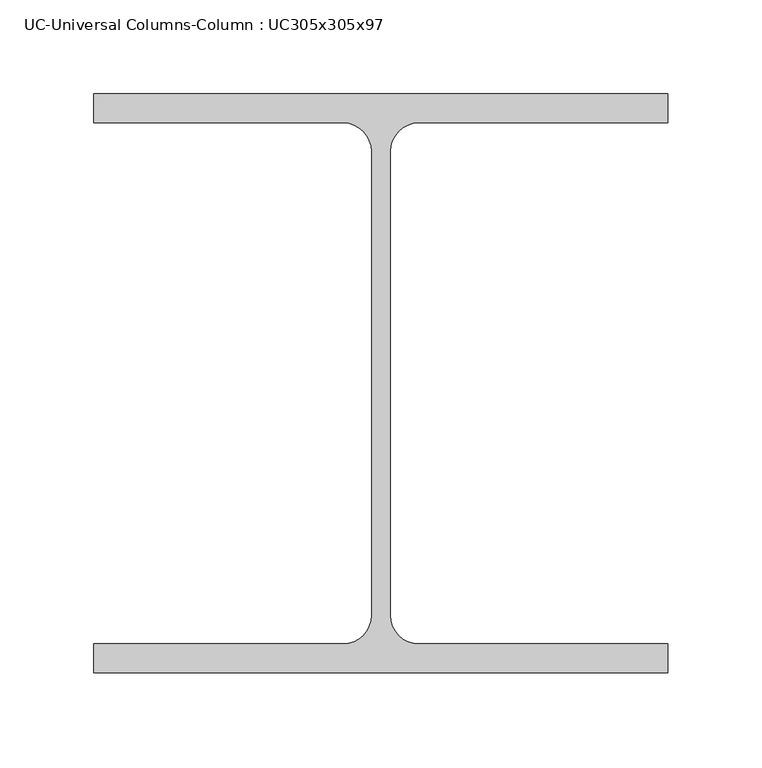
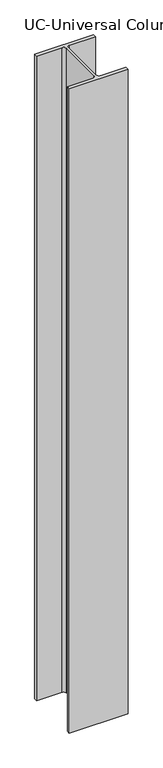
"""IFC4 building model written with IfcOpenShell, lengths in millimetres: column geometry, UC-Universal Columns-Column : UC305x305x97."""

from ifc_helpers import new_model, si_unit, point, frame_2d, origin, origin_with_axes, place, context, project, spatial, polyline, circle_curve, trimmed, segment, composite_curve, outline, extrude, source, transform, mapped, element, save


def uc_universal_columns_column_uc305x305x97_78c6f2b7(model_context):
    return source(origin(), model_context, "Body", "SweptSolid", [
        extrude(outline(composite_curve([segment(polyline([(152.65, -153.95), (-152.65, -153.95), (-152.65, -138.55), (-20.15, -138.55)]), True, "CONTINUOUS"), segment(trimmed(circle_curve(frame_2d((-20.15, -123.35)), 15.2), [point((-20.15, -138.55))], [point((-4.95, -123.35))], True, "CARTESIAN"), True, "CONTINUOUS"), segment(polyline([(-4.95, -123.35), (-4.95, 123.35)]), True, "CONTINUOUS"), segment(trimmed(circle_curve(frame_2d((-20.15, 123.35)), 15.2), [point((-4.95, 123.35))], [point((-20.15, 138.55))], True, "CARTESIAN"), True, "CONTINUOUS"), segment(polyline([(-20.15, 138.55), (-152.65, 138.55), (-152.65, 153.95), (152.65, 153.95), (152.65, 138.55), (20.15, 138.55)]), True, "CONTINUOUS"), segment(trimmed(circle_curve(frame_2d((20.15, 123.35)), 15.2), [point((20.15, 138.55))], [point((4.95, 123.35))], True, "CARTESIAN"), True, "CONTINUOUS"), segment(polyline([(4.95, 123.35), (4.95, -123.35)]), True, "CONTINUOUS"), segment(trimmed(circle_curve(frame_2d((20.15, -123.35)), 15.2), [point((4.95, -123.35))], [point((20.15, -138.55))], True, "CARTESIAN"), True, "CONTINUOUS"), segment(polyline([(20.15, -138.55), (152.65, -138.55), (152.65, -153.95)]), True, "CONTINUOUS")], self_intersect=False)), origin_with_axes(), (0.0, 0.0, 1.0), 3530.0),
    ])


if __name__ == "__main__":
    model = new_model("IFC4")
    model_context = context("Model", 3, world=origin())
    ifc_project = project(units=[si_unit("LENGTHUNIT", "METRE", prefix="MILLI")], contexts=[model_context])
    site = spatial("IfcSite", under=ifc_project)
    building = spatial("IfcBuilding", under=site)
    placement = place(None, origin())
    uc_universal_columns_column_uc305x305x97_shape = uc_universal_columns_column_uc305x305x97_78c6f2b7(model_context)
    element("IfcColumn", 1, ObjectType="UC-Universal Columns-Column : UC305x305x97", at=placement, inside=building, context=model_context, shape_type="MappedRepresentation", body=[
        mapped(uc_universal_columns_column_uc305x305x97_shape, transform((0.0, 0.0, 0.0), x_axis=(1.0, 0.0, 0.0), y_axis=(0.0, 1.0, 0.0), z_axis=(0.0, 0.0, 1.0))),
    ])
    save(model, "model.ifc")

# Revit data of these elements
# Type "UC-Universal Columns-Column : UC305x305x97"
#   Section Name Key = "UC305x305x97"
#   Width = 30.53 cm
#   Web Thickness = 0.99 cm
#   Web Fillet = 1.52 cm
#   Warping Constant = 1560000.0 cm⁶
#   Torsional Moment of Inertia = 91.20 cm⁴
#   Section Area = 123.0 cm²
#   Plastic Modulus weak axis = 726.0 cm³
#   Plastic Modulus strong axis = 1592.0 cm³
#   Nominal Weight = 96.8996 kgf/m
#   Moment of Inertia weak axis = 7308.00 cm⁴
#   Moment of Inertia strong axis = 22249.00 cm⁴
#   Height = 30.79 cm
#   Flange Thickness = 1.54 cm
#   Elastic Modulus weak axis = 479.0 cm³
#   Elastic Modulus strong axis = 1445.0 cm³
#   Centroid Vertical = 15.395 cm
#   Centroid Horizontal = 15.265 cm
#   Bolt Spacing = 14.0 cm
#   Structural Material [instance default] = Metal - Steel 43-275
#   Type Comments = ""
#   Assembly Code = ""
# Element 1 (IfcColumn, "UC-Universal Columns-Column : UC305x305x97")
#   Materials on its faces: "Metal - Steel 43-275"
# Materials
#   "Metal - Steel 43-275": class "Metal", colour RGB 247 247 247, transparency 0, Cost = 0
